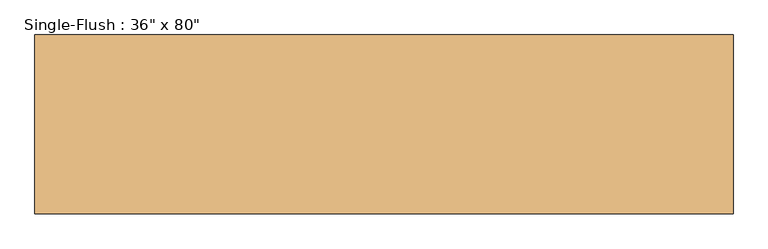
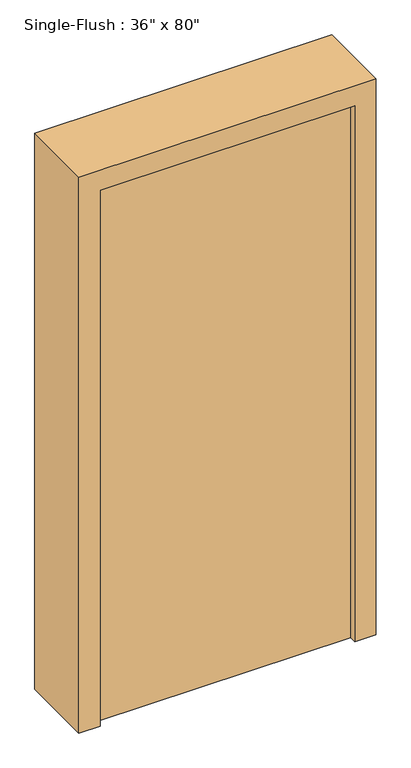
"""IFC4 building model written with IfcOpenShell, lengths in millimetres: door geometry."""

from ifc_helpers import new_model, si_unit, frame, origin, origin_with_axes, place, context, project, spatial, polyline, outline, extrude, source, transform, mapped, element, save


def door_43fbab3f(model_context):
    return source(origin(), model_context, "Body", "SweptSolid", [
        extrude(outline(polyline([(2108.2, 533.4), (2108.2, -533.4), (0.0, -533.4), (0.0, -457.2), (2032.0, -457.2), (2032.0, 457.2), (0.0, 457.2), (0.0, 533.4), (2108.2, 533.4)])), frame((0.0, -136.525, 0.0), z_axis=(0.0, 1.0, 0.0), x_axis=(0.0, 0.0, 1.0)), (0.0, 0.0, 1.0), 273.05),
        extrude(outline(polyline([(457.2, -60.325), (457.2, -111.125), (-457.2, -111.125), (-457.2, -60.325), (457.2, -60.325)])), origin_with_axes(), (0.0, 0.0, 1.0), 2032.0),
    ])


if __name__ == "__main__":
    model = new_model("IFC4")
    model_context = context("Model", 3, world=origin())
    ifc_project = project(units=[si_unit("LENGTHUNIT", "METRE", prefix="MILLI")], contexts=[model_context])
    site = spatial("IfcSite", under=ifc_project)
    building = spatial("IfcBuilding", under=site)
    placement = place(None, origin())
    door_shape = door_43fbab3f(model_context)
    element("IfcDoor", 1, ObjectType="Single-Flush : 36\" x 80\"", at=placement, inside=building, context=model_context, shape_type="MappedRepresentation", body=[
        mapped(door_shape, transform((0.0, 0.0, 0.0), x_axis=(1.0, 0.0, 0.0), y_axis=(0.0, 1.0, 0.0), z_axis=(0.0, 0.0, 1.0))),
    ])
    save(model, "model.ifc")

# Revit data of these elements
# Type "Single-Flush : 36\" x 80\""
#   Type Mark = "13"
#   Construction Type Id = "MDOOR"
#   Assembly Code = "C1020"
#   Analytic Construction = "Metal"
#   Thickness = 0' - 2"
#   Thermal Resistance (R) = 0.270117 (m²·K)/W
#   Heat Transfer Coefficient (U) = 3.7021 W/(m²·K)
#   Height = 6' - 8"
#   Trim Projection Ext = 0' - 1"
#   Trim Projection Int = 0' - 1"
#   Trim Width = 0' - 3"
#   Width = 3' - 0"
#   Door Material = INTERIOR GRADE ALUMINUM STOREFRONT W/ SAFETY GLAZING
#   Frame Material = INTERIOR GRADE ALUMINUM STOREFRONT W/ SAFETY GLAZING
#   Visual Light Transmittance = 0
#   Solar Heat Gain Coefficient = 0
#   Function = (empty or 0)
#   Wall Closure = (empty or 0)
# Element 1 (IfcDoor, "Single-Flush : 36\" x 80\"")
#   Materials on its faces: "INTERIOR GRADE ALUMINUM STOREFRONT W/ SAFETY GLAZING"
# Materials
#   "INTERIOR GRADE ALUMINUM STOREFRONT W/ SAFETY GLAZING": class "Metal", colour RGB 226 226 226, transparency 0, Description = "Aluminum 6061", Cost = 0
